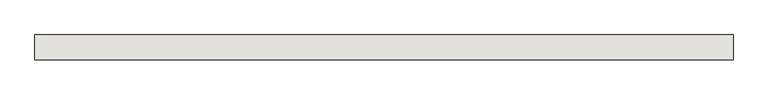
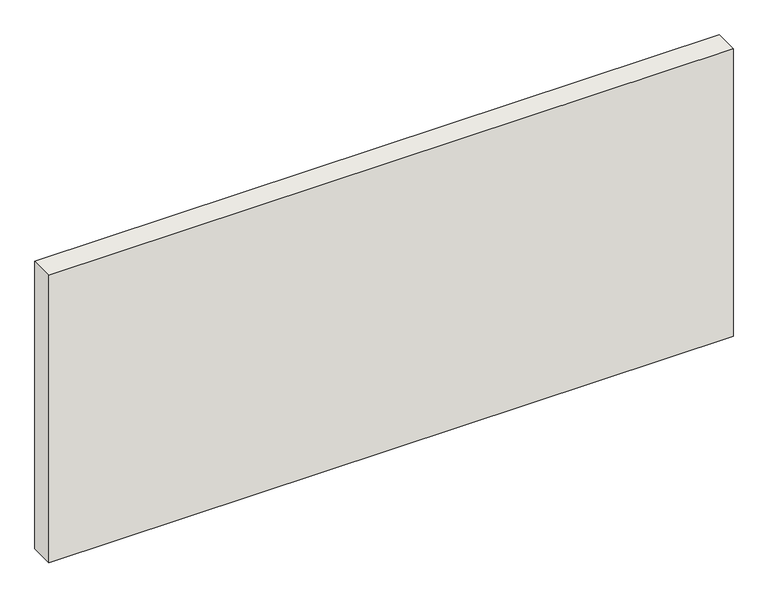
"""IFC4 building model written with IfcOpenShell, lengths in millimetres: wall geometry, Holzwand."""

from ifc_helpers import new_model, si_unit, origin, origin_with_axes, place, context, project, spatial, polyline, outline, extrude, source, transform, mapped, element, save


def wall_fe2e87f2(model_context):
    return source(origin(), model_context, "Body", "SweptSolid", [
        extrude(outline(polyline([(0.0, 200.0), (5650.0, 200.0), (5650.0, 0.0), (0.0, 0.0), (0.0, 200.0)])), origin_with_axes(), (0.0, 0.0, 1.0), 2510.0),
    ])


if __name__ == "__main__":
    model = new_model("IFC4")
    model_context = context("Model", 3, world=origin())
    ifc_project = project(units=[si_unit("LENGTHUNIT", "METRE", prefix="MILLI")], contexts=[model_context])
    site = spatial("IfcSite", under=ifc_project)
    building = spatial("IfcBuilding", under=site)
    placement = place(None, origin())
    wall_shape = wall_fe2e87f2(model_context)
    element("IfcWall", 1, ObjectType="Holzwand", at=placement, inside=building, context=model_context, shape_type="MappedRepresentation", body=[
        mapped(wall_shape, transform((0.0, 0.0, 0.0), x_axis=(1.0, 0.0, 0.0), y_axis=(0.0, 1.0, 0.0), z_axis=(0.0, 0.0, 1.0))),
    ])
    save(model, "model.ifc")

# Revit data of these elements
# Element 1 (IfcWall, "Holzwand")
#   Materials on its faces: "holzschalung"
# Materials
#   "holzschalung": class "Unassigned", colour RGB 128 128 128, transparency 0
